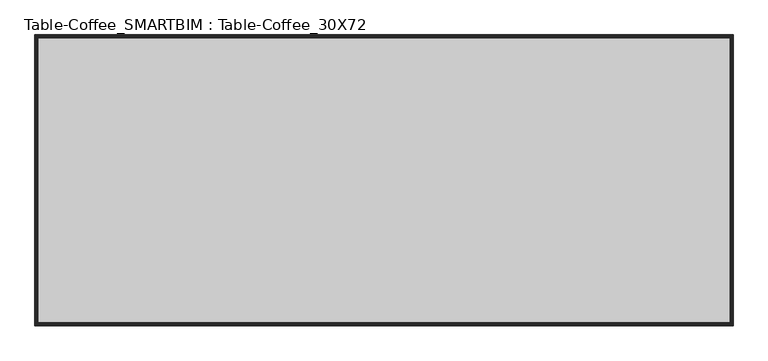
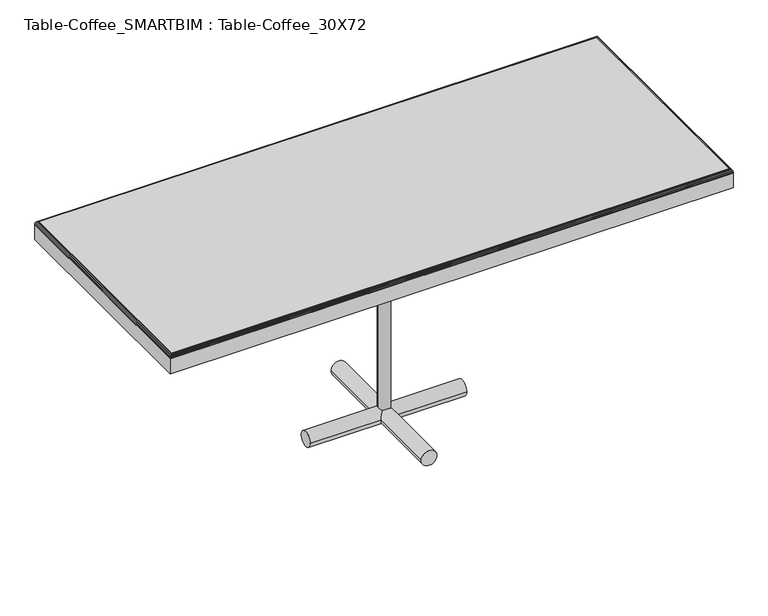
"""IFC4 building model written with IfcOpenShell, lengths in millimetres: furniture geometry, Table-Coffee_SMARTBIM : Table-Coffee_30X72."""

from ifc_helpers import new_model, si_unit, point, frame, frame_2d, origin, origin_2d, place, context, project, spatial, polyline, circle_curve, ellipse_curve, trimmed, segment, composite_curve, outline, extrude, source, transform, mapped, element, save
from ifc_brep_helpers import plane_surface, cylinder_surface, advanced_brep


def table_coffee_smartbim_table_coffee_30x72_ce2343fb(model_context):
    return source(origin(), model_context, "Body", "SolidModel", [
        extrude(outline(composite_curve([segment(trimmed(circle_curve(frame_2d((0.0, 25.4)), 25.4), [point((25.4, 25.4))], [point((-25.4, 25.4))], False, "CARTESIAN"), True, "CONTINUOUS"), segment(trimmed(circle_curve(frame_2d((0.0, 25.4)), 25.4), [point((-25.4, 25.4))], [point((25.4, 25.4))], False, "CARTESIAN"), True, "CONTINUOUS")], self_intersect=False)), frame((-254.0, 0.0, 0.0), z_axis=(1.0, 0.0, 0.0), x_axis=(0.0, 1.0, 0.0)), (0.0, 0.0, 1.0), 508.0),
        extrude(outline(composite_curve([segment(trimmed(circle_curve(frame_2d((25.4, 0.0)), 25.4), [point((25.4, -25.4))], [point((25.4, 25.4))], False, "CARTESIAN"), True, "CONTINUOUS"), segment(trimmed(circle_curve(frame_2d((25.4, 0.0)), 25.4), [point((25.4, 25.4))], [point((25.4, -25.4))], False, "CARTESIAN"), True, "CONTINUOUS")], self_intersect=False)), frame((0.0, -254.0, 0.0), z_axis=(0.0, 1.0, 0.0), x_axis=(0.0, 0.0, 1.0)), (0.0, 0.0, 1.0), 508.0),
        extrude(outline(polyline([(914.4, 381.0), (914.4, -381.0), (-914.4, -381.0), (-914.4, 381.0), (914.4, 381.0)])), frame((0.0, 0.0, 711.2), z_axis=(0.0, 0.0, 1.0), x_axis=(1.0, 0.0, 0.0)), (0.0, 0.0, 1.0), 50.8),
        advanced_brep(
        [(-904.9998654, -371.5998654, 774.7), (904.9998654, -371.5998654, 774.7), (904.9998654, 371.5998654, 774.7), (-904.9998654, 371.5998654, 774.7), (914.4, 381.0, 762.0), (914.4, -381.0, 762.0), (-914.4, -381.0, 762.0), (-914.4, 381.0, 762.0), (-914.4, 381.0, 765.2998654), (914.4, 381.0, 765.2998654), (-914.4, -381.0, 765.2998654), (914.4, -381.0, 765.2998654), (-914.0372483, -380.6372483, 767.8860287), (-914.0372483, 380.6372483, 767.8860287), (-907.1616212, 373.7616212, 774.4480533), (-907.1616212, -373.7616212, 774.4480533), (-909.1639185, 375.7639185, 773.7273912), (-909.1639185, -375.7639185, 773.7273912), (-911.2885738, 377.8885738, 772.2866155), (-911.2885738, -377.8885738, 772.2866155), (-913.3102962, 379.9102962, 769.692959), (-913.3102962, -379.9102962, 769.692959), (914.0372483, -380.6372483, 767.8860287), (907.1616212, -373.7616212, 774.4480533), (909.1639185, -375.7639185, 773.7273912), (911.2885738, -377.8885738, 772.2866155), (913.3102962, -379.9102962, 769.692959), (914.0372483, 380.6372483, 767.8860287), (907.1616212, 373.7616212, 774.4480533), (909.1639185, 375.7639185, 773.7273912), (911.2885738, 377.8885738, 772.2866155), (913.3102962, 379.9102962, 769.692959)],
        [
            (0, 1),
            (1, 2),
            (2, 3),
            (3, 0),
            (4, 5),
            (5, 6),
            (6, 7),
            (7, 4),
            (7, 8),
            (8, 9),
            (9, 4),
            (6, 10),
            (10, 8),
            (5, 11),
            (11, 10),
            (9, 11),
            (10, 12, ellipse_curve(frame((-904.9998654, -371.5998654, 765.2998654), z_axis=(-0.7071067811865475, 0.7071067811865475, 0.0), x_axis=(-0.7071067811865474, -0.7071067811865476, 0.0)), 13.2937978, 9.4001346)),
            (12, 13),
            (13, 8, ellipse_curve(frame((-904.9998654, 371.5998654, 765.2998654), z_axis=(-0.7071067811865475, -0.7071067811865475, 0.0), x_axis=(0.7071067811865474, -0.7071067811865476, 0.0)), 13.2937978, 9.4001346)),
            (14, 15),
            (15, 0, ellipse_curve(frame((-904.9998654, -371.5998654, 765.2998654), z_axis=(-0.7071067811865475, 0.7071067811865475, 0.0), x_axis=(-0.7071067811865474, -0.7071067811865476, 0.0)), 13.2937978, 9.4001346)),
            (3, 14, ellipse_curve(frame((-904.9998654, 371.5998654, 765.2998654), z_axis=(-0.7071067811865475, -0.7071067811865475, 0.0), x_axis=(0.7071067811865474, -0.7071067811865476, 0.0)), 13.2937978, 9.4001346)),
            (14, 16, ellipse_curve(frame((-904.9998654, 371.5998654, 765.2998654), z_axis=(-0.7071067811865475, -0.7071067811865475, 0.0), x_axis=(0.7071067811865474, -0.7071067811865476, 0.0)), 13.2937978, 9.4001346)),
            (16, 17),
            (17, 15, ellipse_curve(frame((-904.9998654, -371.5998654, 765.2998654), z_axis=(-0.7071067811865475, 0.7071067811865475, 0.0), x_axis=(-0.7071067811865474, -0.7071067811865476, 0.0)), 13.2937978, 9.4001346)),
            (16, 18, ellipse_curve(frame((-904.9998654, 371.5998654, 765.2998654), z_axis=(-0.7071067811865475, -0.7071067811865475, 0.0), x_axis=(0.7071067811865474, -0.7071067811865476, 0.0)), 13.2937978, 9.4001346)),
            (18, 19),
            (19, 17, ellipse_curve(frame((-904.9998654, -371.5998654, 765.2998654), z_axis=(-0.7071067811865475, 0.7071067811865475, 0.0), x_axis=(-0.7071067811865474, -0.7071067811865476, 0.0)), 13.2937978, 9.4001346)),
            (18, 20, ellipse_curve(frame((-904.9998654, 371.5998654, 765.2998654), z_axis=(-0.7071067811865475, -0.7071067811865475, 0.0), x_axis=(0.7071067811865474, -0.7071067811865476, 0.0)), 13.2937978, 9.4001346)),
            (20, 21),
            (21, 19, ellipse_curve(frame((-904.9998654, -371.5998654, 765.2998654), z_axis=(-0.7071067811865475, 0.7071067811865475, 0.0), x_axis=(-0.7071067811865474, -0.7071067811865476, 0.0)), 13.2937978, 9.4001346)),
            (12, 21, ellipse_curve(frame((-904.9998654, -371.5998654, 765.2998654), z_axis=(-0.7071067811865475, 0.7071067811865475, 0.0), x_axis=(-0.7071067811865474, -0.7071067811865476, 0.0)), 13.2937978, 9.4001346)),
            (20, 13, ellipse_curve(frame((-904.9998654, 371.5998654, 765.2998654), z_axis=(-0.7071067811865475, -0.7071067811865475, 0.0), x_axis=(0.7071067811865474, -0.7071067811865476, 0.0)), 13.2937978, 9.4001346)),
            (11, 22, ellipse_curve(frame((904.9998654, -371.5998654, 765.2998654), z_axis=(-0.7071067811865475, -0.7071067811865475, 0.0), x_axis=(0.7071067811865476, -0.7071067811865474, 0.0)), 13.2937978, 9.4001346)),
            (22, 12),
            (15, 23),
            (23, 1, ellipse_curve(frame((904.9998654, -371.5998654, 765.2998654), z_axis=(-0.7071067811865475, -0.7071067811865475, 0.0), x_axis=(0.7071067811865476, -0.7071067811865474, 0.0)), 13.2937978, 9.4001346)),
            (17, 24),
            (24, 23, ellipse_curve(frame((904.9998654, -371.5998654, 765.2998654), z_axis=(-0.7071067811865475, -0.7071067811865475, 0.0), x_axis=(0.7071067811865476, -0.7071067811865474, 0.0)), 13.2937978, 9.4001346)),
            (19, 25),
            (25, 24, ellipse_curve(frame((904.9998654, -371.5998654, 765.2998654), z_axis=(-0.7071067811865475, -0.7071067811865475, 0.0), x_axis=(0.7071067811865476, -0.7071067811865474, 0.0)), 13.2937978, 9.4001346)),
            (21, 26),
            (26, 25, ellipse_curve(frame((904.9998654, -371.5998654, 765.2998654), z_axis=(-0.7071067811865475, -0.7071067811865475, 0.0), x_axis=(0.7071067811865476, -0.7071067811865474, 0.0)), 13.2937978, 9.4001346)),
            (22, 26, ellipse_curve(frame((904.9998654, -371.5998654, 765.2998654), z_axis=(-0.7071067811865475, -0.7071067811865475, 0.0), x_axis=(0.7071067811865476, -0.7071067811865474, 0.0)), 13.2937978, 9.4001346)),
            (9, 27, ellipse_curve(frame((904.9998654, 371.5998654, 765.2998654), z_axis=(0.7071067811865475, -0.7071067811865475, 0.0), x_axis=(0.7071067811865474, 0.7071067811865476, 0.0)), 13.2937978, 9.4001346)),
            (27, 22),
            (23, 28),
            (28, 2, ellipse_curve(frame((904.9998654, 371.5998654, 765.2998654), z_axis=(0.7071067811865475, -0.7071067811865475, 0.0), x_axis=(0.7071067811865474, 0.7071067811865476, 0.0)), 13.2937978, 9.4001346)),
            (24, 29),
            (29, 28, ellipse_curve(frame((904.9998654, 371.5998654, 765.2998654), z_axis=(0.7071067811865475, -0.7071067811865475, 0.0), x_axis=(0.7071067811865474, 0.7071067811865476, 0.0)), 13.2937978, 9.4001346)),
            (25, 30),
            (30, 29, ellipse_curve(frame((904.9998654, 371.5998654, 765.2998654), z_axis=(0.7071067811865475, -0.7071067811865475, 0.0), x_axis=(0.7071067811865474, 0.7071067811865476, 0.0)), 13.2937978, 9.4001346)),
            (26, 31),
            (31, 30, ellipse_curve(frame((904.9998654, 371.5998654, 765.2998654), z_axis=(0.7071067811865475, -0.7071067811865475, 0.0), x_axis=(0.7071067811865474, 0.7071067811865476, 0.0)), 13.2937978, 9.4001346)),
            (27, 31, ellipse_curve(frame((904.9998654, 371.5998654, 765.2998654), z_axis=(0.7071067811865475, -0.7071067811865475, 0.0), x_axis=(0.7071067811865474, 0.7071067811865476, 0.0)), 13.2937978, 9.4001346)),
            (13, 27),
            (28, 14),
            (29, 16),
            (30, 18),
            (31, 20),
        ],
        [
            plane_surface(frame((-914.4, 381.0, 774.7), z_axis=(0.0, 0.0, 1.0), x_axis=(-1.0, 0.0, 0.0))),
            plane_surface(frame((-914.4, 381.0, 762.0), z_axis=(0.0, 0.0, -1.0), x_axis=(1.0, 0.0, 0.0))),
            plane_surface(frame((914.4, 381.0, 774.7), z_axis=(0.0, 1.0, 0.0), x_axis=(0.0, 0.0, -1.0))),
            plane_surface(frame((-914.4, 381.0, 774.7), z_axis=(-1.0, 0.0, 0.0), x_axis=(0.0, 0.0, -1.0))),
            plane_surface(frame((-914.4, -381.0, 774.7), z_axis=(0.0, -1.0, 0.0), x_axis=(0.0, 0.0, -1.0))),
            plane_surface(frame((914.4, -381.0, 774.7), z_axis=(1.0, 0.0, 0.0), x_axis=(0.0, 0.0, -1.0))),
            cylinder_surface(frame((-904.9998654, 381.0, 765.2998654), z_axis=(0.0, -1.0, 0.0), x_axis=(1.0, 0.0, 0.0)), 9.4001346),
            cylinder_surface(frame((-914.4, -371.5998654, 765.2998654), z_axis=(1.0, 0.0, 0.0), x_axis=(0.0, 1.0, 0.0)), 9.4001346),
            cylinder_surface(frame((904.9998654, -381.0, 765.2998654), z_axis=(0.0, 1.0, 0.0), x_axis=(-1.0, 0.0, 0.0)), 9.4001346),
            cylinder_surface(frame((914.4, 371.5998654, 765.2998654), z_axis=(-1.0, 0.0, 0.0), x_axis=(0.0, -1.0, 0.0)), 9.4001346),
        ],
        [
            (0, [[1, 2, 3, 4]]),
            (1, [[5, 6, 7, 8]]),
            (2, [[-8, 9, 10, 11]]),
            (3, [[-7, 12, 13, -9]]),
            (4, [[-6, 14, 15, -12]]),
            (5, [[-5, -11, 16, -14]]),
            (6, [[17, 18, 19, -13]]),
            (6, [[20, 21, -4, 22]]),
            (6, [[-20, 23, 24, 25]]),
            (6, [[-24, 26, 27, 28]]),
            (6, [[-27, 29, 30, 31]]),
            (6, [[-18, 32, -30, 33]]),
            (7, [[-17, -15, 34, 35]]),
            (7, [[-21, 36, 37, -1]]),
            (7, [[-25, 38, 39, -36]]),
            (7, [[-28, 40, 41, -38]]),
            (7, [[-31, 42, 43, -40]]),
            (7, [[-32, -35, 44, -42]]),
            (8, [[-34, -16, 45, 46]]),
            (8, [[-37, 47, 48, -2]]),
            (8, [[-39, 49, 50, -47]]),
            (8, [[-41, 51, 52, -49]]),
            (8, [[-43, 53, 54, -51]]),
            (8, [[-44, -46, 55, -53]]),
            (9, [[-19, 56, -45, -10]]),
            (9, [[-22, -3, -48, 57]]),
            (9, [[-23, -57, -50, 58]]),
            (9, [[-26, -58, -52, 59]]),
            (9, [[-29, -59, -54, 60]]),
            (9, [[-33, -60, -55, -56]]),
        ],
    ),
        extrude(outline(polyline([(76.2, 76.2), (76.2, -76.2), (-76.2, -76.2), (-76.2, 76.2), (76.2, 76.2)])), frame((0.0, 0.0, 755.65), z_axis=(0.0, 0.0, 1.0), x_axis=(1.0, 0.0, 0.0)), (0.0, 0.0, 1.0), 6.35),
        extrude(outline(composite_curve([segment(trimmed(circle_curve(origin_2d(), 19.05), [point((-19.05, 0.0))], [point((19.05, 0.0))], False, "CARTESIAN"), True, "CONTINUOUS"), segment(trimmed(circle_curve(origin_2d(), 19.05), [point((19.05, 0.0))], [point((-19.05, 0.0))], False, "CARTESIAN"), True, "CONTINUOUS")], self_intersect=False)), frame((0.0, 0.0, 24.2070278), z_axis=(0.0, 0.0, 1.0), x_axis=(1.0, 0.0, 0.0)), (0.0, 0.0, 1.0), 731.4429722),
    ])


if __name__ == "__main__":
    model = new_model("IFC4")
    model_context = context("Model", 3, world=origin())
    ifc_project = project(units=[si_unit("LENGTHUNIT", "METRE", prefix="MILLI")], contexts=[model_context])
    site = spatial("IfcSite", under=ifc_project)
    building = spatial("IfcBuilding", under=site)
    placement = place(None, origin())
    table_coffee_smartbim_table_coffee_30x72_shape = table_coffee_smartbim_table_coffee_30x72_ce2343fb(model_context)
    element("IfcFurniture", 1, ObjectType="Table-Coffee_SMARTBIM : Table-Coffee_30X72", at=placement, inside=building, context=model_context, shape_type="MappedRepresentation", body=[
        mapped(table_coffee_smartbim_table_coffee_30x72_shape, transform((0.0, 0.0, 0.0), x_axis=(1.0, 0.0, 0.0), y_axis=(0.0, 1.0, 0.0), z_axis=(0.0, 0.0, 1.0))),
    ])
    save(model, "model.ifc")

# Revit data of these elements
# Type "Table-Coffee_SMARTBIM : Table-Coffee_30X72"
#   Subcategory = "Table\r\n"
#   SmartBIM Object Created By = "SMARTBIM, LLC"
#   Manufacturer = "SMARTBIM"
#   Assembly Code = "E2020200"
#   95 CSI = "12500"
#   04 CSI = "12 50 00"
#   table cloth = 0' - 2"
#   Width = 6' - 0"
#   SmartBIM Object Version = 3
#   Height = 2' - 6"
#   Depth = 2' - 6"
#   Default Elevation = 4' - 0"
#   white cloth_parameter = WOOD-OAKFIRE
#   Table Unit = MET
#   Glide = none
#   Glass = none
# Element 1 (IfcFurniture, "Table-Coffee_SMARTBIM : Table-Coffee_30X72")
#   Materials on its faces: "WOOD-OAKFIRE", "MET"
# Materials
#   "WOOD-OAKFIRE": class "Wood", colour RGB 198 202 183, transparency 0, Description = "Generic wood", Cost = 0
#   "MET": class "Metal", colour RGB 189 187 185, transparency 0
